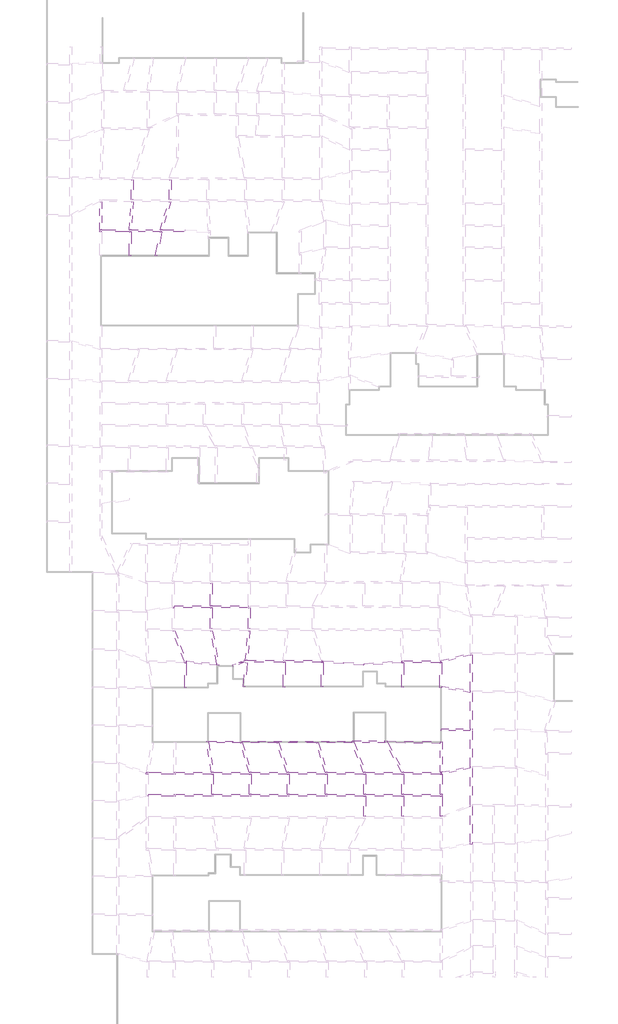
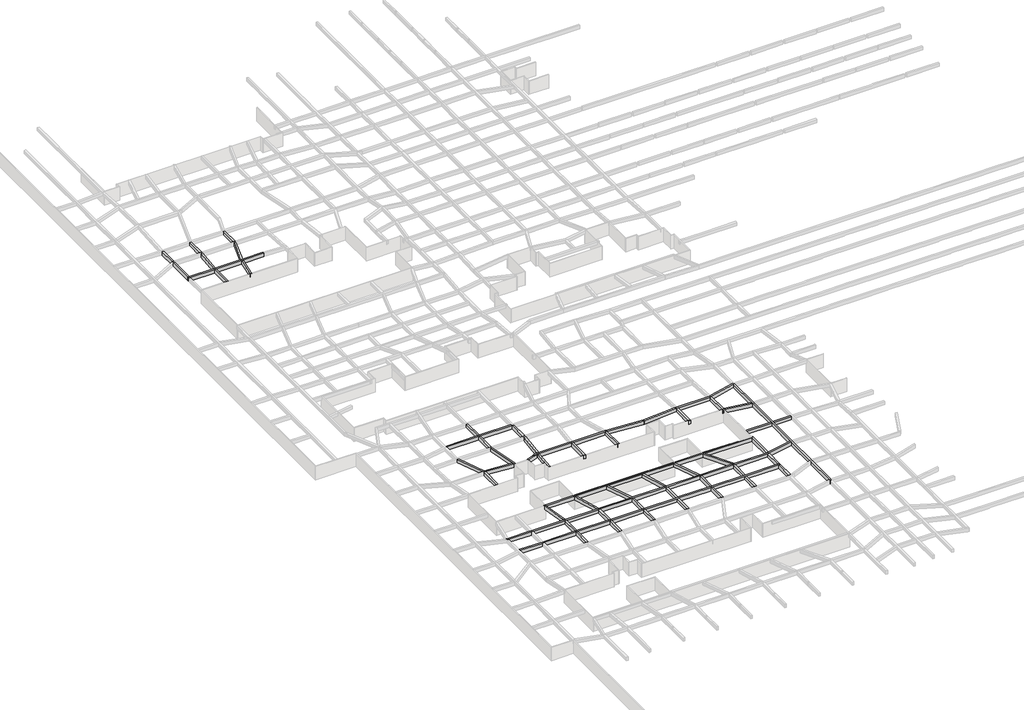
# One storey, part 15 of 45: 55 beams.
"""IFC4 building model written with IfcOpenShell, lengths in millimetres."""

from ifc_helpers import new_model, si_unit, frame, origin, place, context, project, spatial, polyline, outline, extrude, faceted_brep, element, save

model = new_model("IFC4")

# Units and contexts
model_context = context("Model", 3, world=origin())
ifc_project = project(units=[si_unit("LENGTHUNIT", "METRE", prefix="MILLI")], contexts=[model_context])

# Site, building, storey
site = spatial("IfcSite", under=ifc_project)
building = spatial("IfcBuilding", under=site)
storey = spatial("IfcBuildingStorey", under=building, Name="户型图", Elevation=0.0)

# Beams
placement = place(None, origin())
element("IfcBeam", 1, ObjectType="混凝土 - 矩形梁 : KL_beam", at=placement, inside=storey, context=model_context, shape_type="Brep", body=[
    faceted_brep([(-126607.5762912, -9543.8680223, 3300.0), (-126600.5942652, -9143.8680223, 3300.0), (-131304.5883974, -9143.8680223, 3300.0), (-131722.8651, -9143.8680223, 3300.0), (-137689.6115362, -9143.8680223, 3300.0), (-138090.5882954, -9143.8680223, 3300.0), (-143704.0852782, -9143.8680223, 3300.0), (-144104.0852782, -9143.8680223, 3300.0), (-144104.0852782, -9543.8680223, 3300.0), (-143704.0852782, -9543.8680223, 3300.0), (-138104.1004356, -9543.8680223, 3300.0), (-137704.1004356, -9543.8680223, 3300.0), (-131813.2236036, -9543.8680223, 3300.0), (-131407.0529588, -9543.8680223, 3300.0), (-126607.5762912, -9543.8680223, 2500.0), (-144104.0852782, -9543.8680223, 2500.0), (-143704.0852782, -9543.8680223, 2500.0), (-138104.1004356, -9543.8680223, 2500.0), (-137704.1004356, -9543.8680223, 2500.0), (-131813.2236036, -9543.8680223, 2500.0), (-131407.0529588, -9543.8680223, 2500.0), (-126600.5942652, -9143.8680223, 2500.0), (-144104.0852782, -9143.8680223, 2500.0), (-143704.0852782, -9143.8680223, 2500.0), (-138090.5882954, -9143.8680223, 2500.0), (-137689.6115362, -9143.8680223, 2500.0), (-131722.8651, -9143.8680223, 2500.0), (-131304.5883974, -9143.8680223, 2500.0)], [[[0, 1, 2, 3, 4, 5, 6, 7, 8, 9, 10, 11, 12, 13]], [[14, 0, 13, 12, 11, 10, 9, 8, 15, 16, 17, 18, 19, 20]], [[21, 14, 20, 19, 18, 17, 16, 15, 22, 23, 24, 25, 26, 27]], [[1, 21, 27, 26, 25, 24, 23, 22, 7, 6, 5, 4, 3, 2]], [[1, 0, 14, 21]], [[8, 7, 22, 15]]]),
])
element("IfcBeam", 2, ObjectType="混凝土 - 矩形梁 : KL_beam", at=placement, inside=storey, context=model_context, shape_type="Brep", body=[
    faceted_brep([(-143704.0852782, 1228.9879716, 3300.0), (-144104.0852782, 1242.9562794, 3300.0), (-144104.0852782, -2906.533538, 3300.0), (-143704.0852782, -2906.533538, 3300.0), (-143704.0852782, 1193.466462, 3300.0), (-143704.0852782, 1228.9879716, 2500.0), (-143704.0852782, -2906.533538, 2500.0), (-143704.0852782, 1193.466462, 2500.0), (-144104.0852782, 1242.9562794, 2500.0), (-144104.0852782, -2906.533538, 2500.0)], [[[0, 1, 2, 3, 4]], [[5, 0, 4, 3, 6, 7]], [[8, 5, 7, 6, 9]], [[1, 8, 9, 2]], [[1, 0, 5, 8]], [[3, 2, 9, 6]]]),
    faceted_brep([(-143704.0852782, -9143.8680223, 3300.0), (-144104.0852782, -9143.8680223, 3300.0), (-144104.0852782, -9143.8680223, 2500.0), (-143704.0852782, -9143.8680223, 2500.0), (-143704.0852782, -3306.533538, 3300.0), (-144104.0852782, -3306.533538, 3300.0), (-143704.0852782, -3306.533538, 2500.0), (-144104.0852782, -3306.533538, 2500.0)], [[[0, 1, 2, 3]], [[1, 0, 4, 5]], [[0, 3, 6, 4]], [[3, 2, 7, 6]], [[2, 1, 5, 7]], [[5, 4, 6, 7]]]),
])
element("IfcBeam", 3, ObjectType="混凝土 - 矩形梁 : KL_beam", at=placement, inside=storey, context=model_context, shape_type="SweptSolid", body=[
    extrude(outline(polyline([(-137682.4021047, -3306.533538), (-137281.4253454, -3306.533538), (-137689.6115362, -9143.8680223), (-138090.5882954, -9143.8680223), (-137682.4021047, -3306.533538)])), frame((0.0, 0.0, 2500.0), z_axis=(0.0, 0.0, 1.0), x_axis=(1.0, 0.0, 0.0)), (0.0, 0.0, 1.0), 800.0),
])
element("IfcBeam", 4, ObjectType="混凝土 - 矩形梁 : KL_beam", at=placement, inside=storey, context=model_context, shape_type="SweptSolid", body=[
    extrude(outline(polyline([(-137267.9283627, -2906.533538), (-137667.9283627, -2906.533538), (-137667.9283627, 1193.466462), (-137267.9283627, 1193.466462), (-137267.9283627, -2906.533538)])), frame((0.0, 0.0, 2500.0), z_axis=(0.0, 0.0, 1.0), x_axis=(1.0, 0.0, 0.0)), (0.0, 0.0, 1.0), 800.0),
])
element("IfcBeam", 5, ObjectType="混凝土 - 矩形梁 : KL_beam", at=placement, inside=storey, context=model_context, shape_type="SweptSolid", body=[
    extrude(outline(polyline([(-129467.9283627, -2906.533538), (-129867.9283627, -2906.533538), (-129867.9283627, 1193.466462), (-129467.9283627, 1193.466462), (-129467.9283627, -2906.533538)])), frame((0.0, 0.0, 2500.0), z_axis=(0.0, 0.0, 1.0), x_axis=(1.0, 0.0, 0.0)), (0.0, 0.0, 1.0), 800.0),
])
element("IfcBeam", 6, ObjectType="混凝土 - 矩形梁 : KL_beam", at=placement, inside=storey, context=model_context, shape_type="SweptSolid", body=[
    extrude(outline(polyline([(-129938.2128502, -3306.533538), (-129519.9361477, -3306.533538), (-131304.5883974, -9143.8680223), (-131722.8651, -9143.8680223), (-129938.2128502, -3306.533538)])), frame((0.0, 0.0, 2500.0), z_axis=(0.0, 0.0, 1.0), x_axis=(1.0, 0.0, 0.0)), (0.0, 0.0, 1.0), 800.0),
])
element("IfcBeam", 7, ObjectType="混凝土 - 矩形梁 : KL_beam", at=placement, inside=storey, context=model_context, shape_type="SweptSolid", body=[
    extrude(outline(polyline([(-137704.1004356, -14443.9764028), (-138104.1004356, -14443.9764028), (-138104.1004356, -9543.8680223), (-137704.1004356, -9543.8680223), (-137704.1004356, -14443.9764028)])), frame((0.0, 0.0, 2500.0), z_axis=(0.0, 0.0, 1.0), x_axis=(1.0, 0.0, 0.0)), (0.0, 0.0, 1.0), 800.0),
])
element("IfcBeam", 8, ObjectType="混凝土 - 矩形梁 : KL_beam", at=placement, inside=storey, context=model_context, shape_type="SweptSolid", body=[
    extrude(outline(polyline([(-132280.8818583, -14499.5979735), (-132674.8049595, -14430.1387024), (-131813.2236036, -9543.8680223), (-131407.0529588, -9543.8680223), (-132280.8818583, -14499.5979735)])), frame((0.0, 0.0, 2500.0), z_axis=(0.0, 0.0, 1.0), x_axis=(1.0, 0.0, 0.0)), (0.0, 0.0, 1.0), 800.0),
])
element("IfcBeam", 9, ObjectType="混凝土 - 矩形梁 : KL_beam", at=placement, inside=storey, context=model_context, shape_type="SweptSolid", body=[
    extrude(outline(polyline([(-121398.6286131, -81886.7344834), (-120998.6286131, -81886.7344834), (-120998.6286131, -86486.7344834), (-121398.6286131, -86486.7344834), (-121398.6286131, -81886.7344834)])), frame((0.0, 0.0, 2500.0), z_axis=(0.0, 0.0, 1.0), x_axis=(1.0, 0.0, 0.0)), (0.0, 0.0, 1.0), 800.0),
])
element("IfcBeam", 10, ObjectType="混凝土 - 矩形梁 : KL_beam", at=placement, inside=storey, context=model_context, shape_type="Brep", body=[
    faceted_brep([(-73810.3500115, -121175.3373066, 3300.0), (-73848.8656308, -120775.3373066, 3300.0), (-74029.6829415, -120775.3373066, 3300.0), (-81521.8778556, -120775.3373066, 3300.0), (-81979.2194827, -120775.3373066, 3300.0), (-89436.7705689, -120775.3373066, 3300.0), (-89865.2285663, -120775.3373066, 3300.0), (-97325.3650448, -120775.3373066, 3300.0), (-97742.8141387, -120775.3373066, 3300.0), (-105188.5127553, -120775.3373066, 3300.0), (-105613.1046235, -120775.3373066, 3300.0), (-112980.7461054, -120775.3373066, 3300.0), (-113398.1951993, -120775.3373066, 3300.0), (-120758.8698576, -120775.3373066, 3300.0), (-121163.8559079, -120775.3373066, 3300.0), (-128529.6078212, -120775.3373066, 3300.0), (-128929.6078212, -120775.3373066, 3300.0), (-134093.0297116, -120775.3373066, 3300.0), (-134498.6851719, -120775.3373066, 3300.0), (-134529.6078212, -120775.3373066, 3300.0), (-134529.6078212, -120958.5805757, 3300.0), (-134529.6078212, -121118.0480078, 3300.0), (-134529.6078212, -121175.3373066, 3300.0), (-134129.6078212, -121175.3373066, 3300.0), (-128929.6078212, -121175.3373066, 3300.0), (-128529.6078212, -121175.3373066, 3300.0), (-121129.6078212, -121175.3373066, 3300.0), (-120729.6078212, -121175.3373066, 3300.0), (-113329.6078212, -121175.3373066, 3300.0), (-112929.6078212, -121175.3373066, 3300.0), (-105529.6078212, -121175.3373066, 3300.0), (-105129.6078212, -121175.3373066, 3300.0), (-97674.2267606, -121175.3373066, 3300.0), (-97274.2267606, -121175.3373066, 3300.0), (-89774.2267606, -121175.3373066, 3300.0), (-89374.2267606, -121175.3373066, 3300.0), (-81974.2267606, -121175.3373066, 3300.0), (-81574.2267606, -121175.3373066, 3300.0), (-74074.2267606, -121175.3373066, 3300.0), (-73810.3500115, -121175.3373066, 2500.0), (-134529.6078212, -121175.3373066, 2500.0), (-134129.6078212, -121175.3373066, 2500.0), (-128929.6078212, -121175.3373066, 2500.0), (-128529.6078212, -121175.3373066, 2500.0), (-121129.6078212, -121175.3373066, 2500.0), (-120729.6078212, -121175.3373066, 2500.0), (-113329.6078212, -121175.3373066, 2500.0), (-112929.6078212, -121175.3373066, 2500.0), (-105529.6078212, -121175.3373066, 2500.0), (-105129.6078212, -121175.3373066, 2500.0), (-97674.2267606, -121175.3373066, 2500.0), (-97274.2267606, -121175.3373066, 2500.0), (-89774.2267606, -121175.3373066, 2500.0), (-89374.2267606, -121175.3373066, 2500.0), (-81974.2267606, -121175.3373066, 2500.0), (-81574.2267606, -121175.3373066, 2500.0), (-74074.2267606, -121175.3373066, 2500.0), (-73848.8656308, -120775.3373066, 2500.0), (-134529.6078212, -121118.0480078, 2500.0), (-134529.6078212, -120958.5805757, 2500.0), (-134529.6078212, -120775.3373066, 2500.0), (-134498.6851719, -120775.3373066, 2500.0), (-134093.0297116, -120775.3373066, 2500.0), (-128929.6078212, -120775.3373066, 2500.0), (-128529.6078212, -120775.3373066, 2500.0), (-121163.8559079, -120775.3373066, 2500.0), (-120758.8698576, -120775.3373066, 2500.0), (-113398.1951993, -120775.3373066, 2500.0), (-112980.7461054, -120775.3373066, 2500.0), (-105613.1046235, -120775.3373066, 2500.0), (-105188.5127553, -120775.3373066, 2500.0), (-97742.8141387, -120775.3373066, 2500.0), (-97325.3650448, -120775.3373066, 2500.0), (-89865.2285663, -120775.3373066, 2500.0), (-89436.7705689, -120775.3373066, 2500.0), (-81979.2194827, -120775.3373066, 2500.0), (-81521.8778556, -120775.3373066, 2500.0), (-74029.6829415, -120775.3373066, 2500.0)], [[[0, 1, 2, 3, 4, 5, 6, 7, 8, 9, 10, 11, 12, 13, 14, 15, 16, 17, 18, 19, 20, 21, 22, 23, 24, 25, 26, 27, 28, 29, 30, 31, 32, 33, 34, 35, 36, 37, 38]], [[39, 0, 38, 37, 36, 35, 34, 33, 32, 31, 30, 29, 28, 27, 26, 25, 24, 23, 22, 40, 41, 42, 43, 44, 45, 46, 47, 48, 49, 50, 51, 52, 53, 54, 55, 56]], [[57, 39, 56, 55, 54, 53, 52, 51, 50, 49, 48, 47, 46, 45, 44, 43, 42, 41, 40, 58, 59, 60, 61, 62, 63, 64, 65, 66, 67, 68, 69, 70, 71, 72, 73, 74, 75, 76, 77]], [[1, 57, 77, 76, 75, 74, 73, 72, 71, 70, 69, 68, 67, 66, 65, 64, 63, 62, 61, 60, 19, 18, 17, 16, 15, 14, 13, 12, 11, 10, 9, 8, 7, 6, 5, 4, 3, 2]], [[22, 21, 20, 19, 60, 59, 58, 40]], [[1, 0, 39, 57]]]),
])
element("IfcBeam", 11, ObjectType="混凝土 - 矩形梁 : KL_beam", at=placement, inside=storey, context=model_context, shape_type="Brep", body=[
    faceted_brep([(-73674.2267606, -125746.3030805, 3300.0), (-73674.2267606, -125346.3030805, 3300.0), (-74074.2267606, -125346.3030805, 3300.0), (-81574.2267606, -125346.3030805, 3300.0), (-81974.2267606, -125346.3030805, 3300.0), (-89374.2267606, -125346.3030805, 3300.0), (-89774.2267606, -125346.3030805, 3300.0), (-97274.2267606, -125346.3030805, 3300.0), (-97674.2267606, -125346.3030805, 3300.0), (-105129.6078212, -125346.3030805, 3300.0), (-105529.6078212, -125346.3030805, 3300.0), (-112929.6078212, -125346.3030805, 3300.0), (-113329.6078212, -125346.3030805, 3300.0), (-120729.6078212, -125346.3030805, 3300.0), (-121129.6078212, -125346.3030805, 3300.0), (-128529.6078212, -125346.3030805, 3300.0), (-128929.6078212, -125346.3030805, 3300.0), (-134129.6078212, -125346.3030805, 3300.0), (-134129.6078212, -125746.3030805, 3300.0), (-128929.6078212, -125746.3030805, 3300.0), (-128529.6078212, -125746.3030805, 3300.0), (-121129.6078212, -125746.3030805, 3300.0), (-120729.6078212, -125746.3030805, 3300.0), (-113329.6078212, -125746.3030805, 3300.0), (-112929.6078212, -125746.3030805, 3300.0), (-105529.6078212, -125746.3030805, 3300.0), (-105129.6078212, -125746.3030805, 3300.0), (-97674.2267606, -125746.3030805, 3300.0), (-97274.2267606, -125746.3030805, 3300.0), (-89774.2267606, -125746.3030805, 3300.0), (-89374.2267606, -125746.3030805, 3300.0), (-81974.2267606, -125746.3030805, 3300.0), (-81574.2267606, -125746.3030805, 3300.0), (-74074.2267606, -125746.3030805, 3300.0), (-73674.2267606, -125746.3030805, 2500.0), (-134129.6078212, -125746.3030805, 2500.0), (-128929.6078212, -125746.3030805, 2500.0), (-128529.6078212, -125746.3030805, 2500.0), (-121129.6078212, -125746.3030805, 2500.0), (-120729.6078212, -125746.3030805, 2500.0), (-113329.6078212, -125746.3030805, 2500.0), (-112929.6078212, -125746.3030805, 2500.0), (-105529.6078212, -125746.3030805, 2500.0), (-105129.6078212, -125746.3030805, 2500.0), (-97674.2267606, -125746.3030805, 2500.0), (-97274.2267606, -125746.3030805, 2500.0), (-89774.2267606, -125746.3030805, 2500.0), (-89374.2267606, -125746.3030805, 2500.0), (-81974.2267606, -125746.3030805, 2500.0), (-81574.2267606, -125746.3030805, 2500.0), (-74074.2267606, -125746.3030805, 2500.0), (-73674.2267606, -125346.3030805, 2500.0), (-134129.6078212, -125346.3030805, 2500.0), (-128929.6078212, -125346.3030805, 2500.0), (-128529.6078212, -125346.3030805, 2500.0), (-121129.6078212, -125346.3030805, 2500.0), (-120729.6078212, -125346.3030805, 2500.0), (-113329.6078212, -125346.3030805, 2500.0), (-112929.6078212, -125346.3030805, 2500.0), (-105529.6078212, -125346.3030805, 2500.0), (-105129.6078212, -125346.3030805, 2500.0), (-97674.2267606, -125346.3030805, 2500.0), (-97274.2267606, -125346.3030805, 2500.0), (-89774.2267606, -125346.3030805, 2500.0), (-89374.2267606, -125346.3030805, 2500.0), (-81974.2267606, -125346.3030805, 2500.0), (-81574.2267606, -125346.3030805, 2500.0), (-74074.2267606, -125346.3030805, 2500.0)], [[[0, 1, 2, 3, 4, 5, 6, 7, 8, 9, 10, 11, 12, 13, 14, 15, 16, 17, 18, 19, 20, 21, 22, 23, 24, 25, 26, 27, 28, 29, 30, 31, 32, 33]], [[34, 0, 33, 32, 31, 30, 29, 28, 27, 26, 25, 24, 23, 22, 21, 20, 19, 18, 35, 36, 37, 38, 39, 40, 41, 42, 43, 44, 45, 46, 47, 48, 49, 50]], [[51, 34, 50, 49, 48, 47, 46, 45, 44, 43, 42, 41, 40, 39, 38, 37, 36, 35, 52, 53, 54, 55, 56, 57, 58, 59, 60, 61, 62, 63, 64, 65, 66, 67]], [[1, 51, 67, 66, 65, 64, 63, 62, 61, 60, 59, 58, 57, 56, 55, 54, 53, 52, 17, 16, 15, 14, 13, 12, 11, 10, 9, 8, 7, 6, 5, 4, 3, 2]], [[18, 17, 52, 35]], [[1, 0, 34, 51]]]),
])
element("IfcBeam", 12, ObjectType="混凝土 - 矩形梁 : KL_beam", at=placement, inside=storey, context=model_context, shape_type="SweptSolid", body=[
    extrude(outline(polyline([(-121129.6078212, -121175.3373066), (-120729.6078212, -121175.3373066), (-120729.6078212, -125346.3030805), (-121129.6078212, -125346.3030805), (-121129.6078212, -121175.3373066)])), frame((0.0, 0.0, 2500.0), z_axis=(0.0, 0.0, 1.0), x_axis=(1.0, 0.0, 0.0)), (0.0, 0.0, 1.0), 800.0),
    extrude(outline(polyline([(-120729.6078212, -129869.3244435), (-121129.6078212, -129869.3244435), (-121129.6078212, -125746.3030805), (-120729.6078212, -125746.3030805), (-120729.6078212, -129869.3244435)])), frame((0.0, 0.0, 2500.0), z_axis=(0.0, 0.0, 1.0), x_axis=(1.0, 0.0, 0.0)), (0.0, 0.0, 1.0), 800.0),
])
element("IfcBeam", 13, ObjectType="混凝土 - 矩形梁 : KL_beam", at=placement, inside=storey, context=model_context, shape_type="SweptSolid", body=[
    extrude(outline(polyline([(-113329.6078212, -121175.3373066), (-112929.6078212, -121175.3373066), (-112929.6078212, -125346.3030805), (-113329.6078212, -125346.3030805), (-113329.6078212, -121175.3373066)])), frame((0.0, 0.0, 2500.0), z_axis=(0.0, 0.0, 1.0), x_axis=(1.0, 0.0, 0.0)), (0.0, 0.0, 1.0), 800.0),
    extrude(outline(polyline([(-112929.6078212, -129869.3244435), (-113329.6078212, -129869.3244435), (-113329.6078212, -125746.3030805), (-112929.6078212, -125746.3030805), (-112929.6078212, -129869.3244435)])), frame((0.0, 0.0, 2500.0), z_axis=(0.0, 0.0, 1.0), x_axis=(1.0, 0.0, 0.0)), (0.0, 0.0, 1.0), 800.0),
])
element("IfcBeam", 14, ObjectType="混凝土 - 矩形梁 : KL_beam", at=placement, inside=storey, context=model_context, shape_type="SweptSolid", body=[
    extrude(outline(polyline([(-105529.6078212, -121175.3373066), (-105129.6078212, -121175.3373066), (-105129.6078212, -125346.3030805), (-105529.6078212, -125346.3030805), (-105529.6078212, -121175.3373066)])), frame((0.0, 0.0, 2500.0), z_axis=(0.0, 0.0, 1.0), x_axis=(1.0, 0.0, 0.0)), (0.0, 0.0, 1.0), 800.0),
    extrude(outline(polyline([(-105129.6078212, -129869.3244435), (-105529.6078212, -129869.3244435), (-105529.6078212, -125746.3030805), (-105129.6078212, -125746.3030805), (-105129.6078212, -129869.3244435)])), frame((0.0, 0.0, 2500.0), z_axis=(0.0, 0.0, 1.0), x_axis=(1.0, 0.0, 0.0)), (0.0, 0.0, 1.0), 800.0),
])
element("IfcBeam", 15, ObjectType="混凝土 - 矩形梁 : KL_beam", at=placement, inside=storey, context=model_context, shape_type="Brep", body=[
    faceted_brep([(-113598.6286131, -86886.7344834, 3300.0), (-113598.6286131, -86486.7344834, 3300.0), (-120998.6286131, -86486.7344834, 3300.0), (-121398.6286131, -86486.7344834, 3300.0), (-128818.6286131, -86486.7344834, 3300.0), (-128818.6286131, -86854.5544096, 3300.0), (-129001.1308804, -86886.7344834, 3300.0), (-128818.6286131, -86886.7344834, 3300.0), (-121398.6286131, -86886.7344834, 3300.0), (-120998.6286131, -86886.7344834, 3300.0), (-113598.6286131, -86886.7344834, 2500.0), (-129001.1308804, -86886.7344834, 2500.0), (-128818.6286131, -86886.7344834, 2500.0), (-121398.6286131, -86886.7344834, 2500.0), (-120998.6286131, -86886.7344834, 2500.0), (-113598.6286131, -86486.7344834, 2500.0), (-128818.6286131, -86854.5544096, 2500.0), (-128818.6286131, -86486.7344834, 2500.0), (-121398.6286131, -86486.7344834, 2500.0), (-120998.6286131, -86486.7344834, 2500.0)], [[[0, 1, 2, 3, 4, 5, 6, 7, 8, 9]], [[10, 0, 9, 8, 7, 6, 11, 12, 13, 14]], [[15, 10, 14, 13, 12, 11, 16, 17, 18, 19]], [[1, 15, 19, 18, 17, 4, 3, 2]], [[1, 0, 10, 15]], [[16, 5, 4, 17]], [[5, 16, 11, 6]]]),
])
element("IfcBeam", 16, ObjectType="混凝土 - 矩形梁 : KL_beam", at=placement, inside=storey, context=model_context, shape_type="SweptSolid", body=[
    extrude(outline(polyline([(-121398.6286131, -86886.7344834), (-120998.6286131, -86886.7344834), (-120998.6286131, -91241.7669719), (-121398.6286131, -91241.7669719), (-121398.6286131, -86886.7344834)])), frame((0.0, 0.0, 2500.0), z_axis=(0.0, 0.0, 1.0), x_axis=(1.0, 0.0, 0.0)), (0.0, 0.0, 1.0), 800.0),
])
element("IfcBeam", 17, ObjectType="混凝土 - 矩形梁 : KL_beam", at=placement, inside=storey, context=model_context, shape_type="Brep", body=[
    faceted_brep([(-126624.1724793, -98237.624084, 3300.0), (-126600.2797743, -98228.4525338, 3300.0), (-126250.7403087, -98094.2769042, 3300.0), (-126344.786832, -97849.2773349, 3300.0), (-128727.6268074, -91641.7669719, 3300.0), (-129156.0848049, -91641.7669719, 3300.0), (-126777.7180933, -97837.624084, 3300.0), (-126624.1724793, -98237.624084, 2500.0), (-129156.0848049, -91641.7669719, 2500.0), (-126777.7180933, -97837.624084, 2500.0), (-126250.7403087, -98094.2769042, 2500.0), (-126600.2797743, -98228.4525338, 2500.0), (-128727.6268074, -91641.7669719, 2500.0), (-126344.786832, -97849.2773349, 2500.0)], [[[0, 1, 2, 3, 4, 5, 6]], [[7, 0, 6, 5, 8, 9]], [[10, 11, 7, 9, 8, 12, 13]], [[2, 10, 13, 12, 4, 3]], [[5, 4, 12, 8]], [[2, 1, 0, 7, 11, 10]]]),
])
element("IfcBeam", 18, ObjectType="混凝土 - 矩形梁 : KL_beam", at=placement, inside=storey, context=model_context, shape_type="Brep", body=[
    faceted_brep([(-119970.4261366, -98808.4895679, 3300.0), (-119577.7752632, -98732.1659698, 3300.0), (-120956.0092123, -91641.7669719, 3300.0), (-121363.4958903, -91641.7669719, 3300.0), (-120049.8255327, -98400.0150859, 3300.0), (-119970.4261366, -98808.4895679, 2500.0), (-121363.4958903, -91641.7669719, 2500.0), (-120049.8255327, -98400.0150859, 2500.0), (-119577.7752632, -98732.1659698, 2500.0), (-120956.0092123, -91641.7669719, 2500.0)], [[[0, 1, 2, 3, 4]], [[5, 0, 4, 3, 6, 7]], [[8, 5, 7, 6, 9]], [[1, 8, 9, 2]], [[3, 2, 9, 6]], [[1, 0, 5, 8]]]),
])
element("IfcBeam", 19, ObjectType="混凝土 - 矩形梁 : KL_beam", at=placement, inside=storey, context=model_context, shape_type="Brep", body=[
    faceted_brep([(-98302.2751608, -98176.6407423, 3300.0), (-98287.4686336, -97776.6407423, 3300.0), (-98563.7893521, -97776.6407423, 3300.0), (-105946.1060855, -97776.6407423, 3300.0), (-106347.6340205, -97776.6407423, 3300.0), (-113752.0942854, -97776.6407423, 3300.0), (-114153.6222204, -97776.6407423, 3300.0), (-114450.8945963, -97776.6407423, 3300.0), (-115492.9302222, -98176.6407423, 3300.0), (-114376.7589783, -98176.6407423, 3300.0), (-106364.3677857, -98176.6407423, 3300.0), (-105964.3677857, -98176.6407423, 3300.0), (-98494.8718972, -98176.6407423, 3300.0), (-98287.4686336, -97776.6407423, 2500.0), (-98563.7893521, -97776.6407423, 2500.0), (-105946.1060855, -97776.6407423, 2500.0), (-106347.6340205, -97776.6407423, 2500.0), (-113752.0942854, -97776.6407423, 2500.0), (-114153.6222204, -97776.6407423, 2500.0), (-114450.8945963, -97776.6407423, 2500.0), (-98302.2751608, -98176.6407423, 2500.0), (-98494.8718972, -98176.6407423, 2500.0), (-105964.3677857, -98176.6407423, 2500.0), (-106364.3677857, -98176.6407423, 2500.0), (-114376.7589783, -98176.6407423, 2500.0), (-115492.9302222, -98176.6407423, 2500.0)], [[[0, 1, 2, 3, 4, 5, 6, 7, 8, 9, 10, 11, 12]], [[1, 13, 14, 15, 16, 17, 18, 19, 7, 6, 5, 4, 3, 2]], [[13, 20, 21, 22, 23, 24, 25, 19, 18, 17, 16, 15, 14]], [[20, 0, 12, 11, 10, 9, 8, 25, 24, 23, 22, 21]], [[0, 20, 13, 1]], [[8, 7, 19, 25]]]),
])
element("IfcBeam", 20, ObjectType="混凝土 - 矩形梁 : KL_beam", at=placement, inside=storey, context=model_context, shape_type="Brep", body=[
    faceted_brep([(-73955.7721969, -98206.5978244, 3300.0), (-74005.7852131, -97806.5978244, 3300.0), (-74190.6863209, -97806.5978244, 3300.0), (-81590.2186825, -97806.5978244, 3300.0), (-81990.6863209, -97806.5978244, 3300.0), (-81989.968125, -97821.4460968, 3300.0), (-81980.778705, -98011.431897, 3300.0), (-81971.3387275, -98206.5978244, 3300.0), (-81580.778705, -98206.5978244, 3300.0), (-74180.6241203, -98206.5978244, 3300.0), (-73955.7721969, -98206.5978244, 2500.0), (-81971.3387275, -98206.5978244, 2500.0), (-81580.778705, -98206.5978244, 2500.0), (-74180.6241203, -98206.5978244, 2500.0), (-74005.7852131, -97806.5978244, 2500.0), (-81980.778705, -98011.431897, 2500.0), (-81989.968125, -97821.4460968, 2500.0), (-81990.6863209, -97806.5978244, 2500.0), (-81590.2186825, -97806.5978244, 2500.0), (-74190.6863209, -97806.5978244, 2500.0)], [[[0, 1, 2, 3, 4, 5, 6, 7, 8, 9]], [[10, 0, 9, 8, 7, 11, 12, 13]], [[14, 10, 13, 12, 11, 15, 16, 17, 18, 19]], [[1, 14, 19, 18, 17, 4, 3, 2]], [[1, 0, 10, 14]], [[7, 6, 5, 4, 17, 16, 15, 11]]]),
])
element("IfcBeam", 21, ObjectType="混凝土 - 矩形梁 : KL_beam", at=placement, inside=storey, context=model_context, shape_type="Brep", body=[
    faceted_brep([(-67725.9320986, -96211.286122, 3300.0), (-67830.7823984, -96237.9219218, 3300.0), (-73792.8353015, -97752.5007811, 3300.0), (-74005.7852131, -97806.5978244, 3300.0), (-73955.7721969, -98206.5978244, 3300.0), (-73780.6241203, -98162.1038257, 3300.0), (-67830.7823984, -96650.6270517, 3300.0), (-67675.9190824, -96611.286122, 3300.0), (-73955.7721969, -98206.5978244, 2500.0), (-73780.6241203, -98162.1038257, 2500.0), (-67830.7823984, -96650.6270517, 2500.0), (-67675.9190824, -96611.286122, 2500.0), (-74005.7852131, -97806.5978244, 2500.0), (-73792.8353015, -97752.5007811, 2500.0), (-67830.7823984, -96237.9219218, 2500.0), (-67725.9320986, -96211.286122, 2500.0)], [[[0, 1, 2, 3, 4, 5, 6, 7]], [[7, 6, 5, 4, 8, 9, 10, 11]], [[11, 10, 9, 8, 12, 13, 14, 15]], [[3, 2, 1, 0, 15, 14, 13, 12]], [[0, 7, 11, 15]], [[3, 12, 8, 4]]]),
])
element("IfcBeam", 22, ObjectType="混凝土 - 矩形梁 : KL_beam", at=placement, inside=storey, context=model_context, shape_type="Brep", body=[
    faceted_brep([(-67430.7823984, -96611.286122, 3300.0), (-67675.9190824, -96611.286122, 3300.0), (-67830.7823984, -96650.6270517, 3300.0), (-67830.7823984, -103977.1522138, 3300.0), (-67830.7823984, -104382.1285271, 3300.0), (-67830.7823984, -111828.4346923, 3300.0), (-67830.7823984, -112228.4346923, 3300.0), (-67830.7823984, -119605.5404275, 3300.0), (-67830.7823984, -120013.0271055, 3300.0), (-67830.7823984, -127430.3404481, 3300.0), (-67830.7823984, -127861.7543451, 3300.0), (-67830.7823984, -135248.1884022, 3300.0), (-67830.7823984, -135656.5378646, 3300.0), (-67764.0267672, -135642.8272555, 3300.0), (-67610.4560354, -135611.286122, 3300.0), (-67430.7823984, -135574.3838418, 3300.0), (-67430.7823984, -135211.286122, 3300.0), (-67430.7823984, -127765.3480623, 3300.0), (-67430.7823984, -127365.3480623, 3300.0), (-67430.7823984, -119970.4077047, 3300.0), (-67430.7823984, -119570.4077047, 3300.0), (-67430.7823984, -112228.4346923, 3300.0), (-67430.7823984, -111828.4346923, 3300.0), (-67430.7823984, -104411.286122, 3300.0), (-67430.7823984, -104011.286122, 3300.0), (-67830.7823984, -96650.6270517, 2500.0), (-67830.7823984, -103977.1522138, 2500.0), (-67830.7823984, -104382.1285271, 2500.0), (-67830.7823984, -111828.4346923, 2500.0), (-67830.7823984, -112228.4346923, 2500.0), (-67830.7823984, -119605.5404275, 2500.0), (-67830.7823984, -120013.0271055, 2500.0), (-67830.7823984, -127430.3404481, 2500.0), (-67830.7823984, -127861.7543451, 2500.0), (-67830.7823984, -135248.1884022, 2500.0), (-67830.7823984, -135656.5378646, 2500.0), (-67675.9190824, -96611.286122, 2500.0), (-67430.7823984, -96611.286122, 2500.0), (-67430.7823984, -104011.286122, 2500.0), (-67430.7823984, -104411.286122, 2500.0), (-67430.7823984, -111828.4346923, 2500.0), (-67430.7823984, -112228.4346923, 2500.0), (-67430.7823984, -119570.4077047, 2500.0), (-67430.7823984, -119970.4077047, 2500.0), (-67430.7823984, -127365.3480623, 2500.0), (-67430.7823984, -127765.3480623, 2500.0), (-67430.7823984, -135211.286122, 2500.0), (-67430.7823984, -135574.3838418, 2500.0), (-67610.4560354, -135611.286122, 2500.0), (-67764.0267672, -135642.8272555, 2500.0)], [[[0, 1, 2, 3, 4, 5, 6, 7, 8, 9, 10, 11, 12, 13, 14, 15, 16, 17, 18, 19, 20, 21, 22, 23, 24]], [[2, 25, 26, 27, 28, 29, 30, 31, 32, 33, 34, 35, 12, 11, 10, 9, 8, 7, 6, 5, 4, 3]], [[36, 37, 38, 39, 40, 41, 42, 43, 44, 45, 46, 47, 48, 49, 35, 34, 33, 32, 31, 30, 29, 28, 27, 26, 25]], [[37, 0, 24, 23, 22, 21, 20, 19, 18, 17, 16, 15, 47, 46, 45, 44, 43, 42, 41, 40, 39, 38]], [[1, 0, 37, 36]], [[2, 1, 36, 25]], [[15, 14, 13, 12, 35, 49, 48, 47]]]),
])
element("IfcBeam", 23, ObjectType="混凝土 - 矩形梁 : KL_beam", at=placement, inside=storey, context=model_context, shape_type="Brep", body=[
    faceted_brep([(-73848.8656308, -120775.3373066, 3300.0), (-73810.3500115, -121175.3373066, 3300.0), (-73674.2267606, -121148.877627, 3300.0), (-67830.7823984, -120013.0271055, 3300.0), (-67830.7823984, -119605.5404275, 3300.0), (-73629.6829415, -120732.7325077, 3300.0), (-73810.3500115, -121175.3373066, 2500.0), (-73674.2267606, -121148.877627, 2500.0), (-67830.7823984, -120013.0271055, 2500.0), (-73848.8656308, -120775.3373066, 2500.0), (-73629.6829415, -120732.7325077, 2500.0), (-67830.7823984, -119605.5404275, 2500.0)], [[[0, 1, 2, 3, 4, 5]], [[1, 6, 7, 8, 3, 2]], [[6, 9, 10, 11, 8, 7]], [[9, 0, 5, 4, 11, 10]], [[0, 9, 6, 1]], [[4, 3, 8, 11]]]),
])
element("IfcBeam", 24, ObjectType="混凝土 - 矩形梁 : KL_beam", at=placement, inside=storey, context=model_context, shape_type="SweptSolid", body=[
    extrude(outline(polyline([(-97674.2267606, -121175.3373066), (-97274.2267606, -121175.3373066), (-97274.2267606, -125346.3030805), (-97674.2267606, -125346.3030805), (-97674.2267606, -121175.3373066)])), frame((0.0, 0.0, 2500.0), z_axis=(0.0, 0.0, 1.0), x_axis=(1.0, 0.0, 0.0)), (0.0, 0.0, 1.0), 800.0),
    extrude(outline(polyline([(-97274.2267606, -129869.3244435), (-97674.2267606, -129869.3244435), (-97674.2267606, -125746.3030805), (-97274.2267606, -125746.3030805), (-97274.2267606, -129869.3244435)])), frame((0.0, 0.0, 2500.0), z_axis=(0.0, 0.0, 1.0), x_axis=(1.0, 0.0, 0.0)), (0.0, 0.0, 1.0), 800.0),
])
element("IfcBeam", 25, ObjectType="混凝土 - 矩形梁 : KL_beam", at=placement, inside=storey, context=model_context, shape_type="Brep", body=[
    faceted_brep([(-91909.5094207, -114333.6323638, 3300.0), (-91968.3714548, -114356.2273817, 3300.0), (-92282.9415913, -114476.9795436, 3300.0), (-92175.7483894, -114756.2273817, 3300.0), (-89865.2285663, -120775.3373066, 3300.0), (-89436.7705689, -120775.3373066, 3300.0), (-91755.9638067, -114733.6323638, 3300.0), (-91909.5094207, -114333.6323638, 2500.0), (-89436.7705689, -120775.3373066, 2500.0), (-91755.9638067, -114733.6323638, 2500.0), (-92282.9415913, -114476.9795436, 2500.0), (-91968.3714548, -114356.2273817, 2500.0), (-89865.2285663, -120775.3373066, 2500.0), (-92175.7483894, -114756.2273817, 2500.0)], [[[0, 1, 2, 3, 4, 5, 6]], [[7, 0, 6, 5, 8, 9]], [[10, 11, 7, 9, 8, 12, 13]], [[2, 10, 13, 12, 4, 3]], [[5, 4, 12, 8]], [[2, 1, 0, 7, 11, 10]]]),
])
element("IfcBeam", 26, ObjectType="混凝土 - 矩形梁 : KL_beam", at=placement, inside=storey, context=model_context, shape_type="Brep", body=[
    faceted_brep([(-85092.5732122, -114333.6323638, 3300.0), (-85549.9148393, -114333.6323638, 3300.0), (-85328.1912188, -114733.6323638, 3300.0), (-81979.2194827, -120775.3373066, 3300.0), (-81521.8778556, -120775.3373066, 3300.0), (-84868.4375117, -114737.9838712, 3300.0), (-85091.7243385, -114335.1637725, 3300.0), (-85092.5732122, -114333.6323638, 2500.0), (-81521.8778556, -120775.3373066, 2500.0), (-84868.4375117, -114737.9838712, 2500.0), (-85091.7243385, -114335.1637725, 2500.0), (-85549.9148393, -114333.6323638, 2500.0), (-81979.2194827, -120775.3373066, 2500.0), (-85328.1912188, -114733.6323638, 2500.0)], [[[0, 1, 2, 3, 4, 5, 6]], [[7, 0, 6, 5, 4, 8, 9, 10]], [[11, 7, 10, 9, 8, 12, 13]], [[1, 11, 13, 12, 3, 2]], [[4, 3, 12, 8]], [[1, 0, 7, 11]]]),
])
element("IfcBeam", 27, ObjectType="混凝土 - 矩形梁 : KL_beam", at=placement, inside=storey, context=model_context, shape_type="Brep", body=[
    faceted_brep([(-74029.6829415, -120775.3373066, 3300.0), (-73848.8656308, -120775.3373066, 3300.0), (-73629.6829415, -120732.7325077, 3300.0), (-73629.6829415, -114478.3270492, 3300.0), (-74029.6829415, -114473.3309662, 3300.0), (-74029.6829415, -114873.362166, 3300.0), (-73629.6829415, -114478.3270492, 2500.0), (-73629.6829415, -120732.7325077, 2500.0), (-73848.8656308, -120775.3373066, 2500.0), (-74029.6829415, -120775.3373066, 2500.0), (-74029.6829415, -114873.362166, 2500.0), (-74029.6829415, -114473.3309662, 2500.0)], [[[0, 1, 2, 3, 4, 5]], [[6, 3, 2, 7]], [[8, 9, 10, 11, 6, 7]], [[9, 0, 5, 4, 11, 10]], [[1, 0, 9, 8]], [[2, 1, 8, 7]], [[4, 3, 6, 11]]]),
])
element("IfcBeam", 28, ObjectType="混凝土 - 矩形梁 : KL_beam", at=placement, inside=storey, context=model_context, shape_type="Brep", body=[
    faceted_brep([(-74074.2267606, -125346.3030805, 3300.0), (-73674.2267606, -125346.3030805, 3300.0), (-73674.2267606, -121148.877627, 3300.0), (-73810.3500115, -121175.3373066, 3300.0), (-74029.6829415, -121175.3373066, 3300.0), (-74074.2267606, -121175.3373066, 3300.0), (-73674.2267606, -125346.3030805, 2500.0), (-73674.2267606, -121148.877627, 2500.0), (-74074.2267606, -125346.3030805, 2500.0), (-74074.2267606, -121175.3373066, 2500.0), (-74029.6829415, -121175.3373066, 2500.0), (-73810.3500115, -121175.3373066, 2500.0)], [[[0, 1, 2, 3, 4, 5]], [[1, 6, 7, 2]], [[6, 8, 9, 10, 11, 7]], [[8, 0, 5, 9]], [[1, 0, 8, 6]], [[9, 5, 4, 3, 11, 10]], [[3, 2, 7, 11]]]),
])
element("IfcBeam", 29, ObjectType="混凝土 - 矩形梁 : KL_beam", at=placement, inside=storey, context=model_context, shape_type="SweptSolid", body=[
    extrude(outline(polyline([(-81974.2267606, -121175.3373066), (-81574.2267606, -121175.3373066), (-81574.2267606, -125346.3030805), (-81974.2267606, -125346.3030805), (-81974.2267606, -121175.3373066)])), frame((0.0, 0.0, 2500.0), z_axis=(0.0, 0.0, 1.0), x_axis=(1.0, 0.0, 0.0)), (0.0, 0.0, 1.0), 800.0),
])
element("IfcBeam", 30, ObjectType="混凝土 - 矩形梁 : KL_beam", at=placement, inside=storey, context=model_context, shape_type="SweptSolid", body=[
    extrude(outline(polyline([(-89774.2267606, -121175.3373066), (-89374.2267606, -121175.3373066), (-89374.2267606, -125346.3030805), (-89774.2267606, -125346.3030805), (-89774.2267606, -121175.3373066)])), frame((0.0, 0.0, 2500.0), z_axis=(0.0, 0.0, 1.0), x_axis=(1.0, 0.0, 0.0)), (0.0, 0.0, 1.0), 800.0),
])
element("IfcBeam", 31, ObjectType="混凝土 - 矩形梁 : KL_beam", at=placement, inside=storey, context=model_context, shape_type="SweptSolid", body=[
    extrude(outline(polyline([(-89774.2267606, -125746.3030805), (-89374.2267606, -125746.3030805), (-89374.2267606, -129869.3244435), (-89774.2267606, -129869.3244435), (-89774.2267606, -125746.3030805)])), frame((0.0, 0.0, 2500.0), z_axis=(0.0, 0.0, 1.0), x_axis=(1.0, 0.0, 0.0)), (0.0, 0.0, 1.0), 800.0),
])
element("IfcBeam", 32, ObjectType="混凝土 - 矩形梁 : KL_beam", at=placement, inside=storey, context=model_context, shape_type="SweptSolid", body=[
    extrude(outline(polyline([(-81974.2267606, -125746.3030805), (-81574.2267606, -125746.3030805), (-81574.2267606, -129869.3244435), (-81974.2267606, -129869.3244435), (-81974.2267606, -125746.3030805)])), frame((0.0, 0.0, 2500.0), z_axis=(0.0, 0.0, 1.0), x_axis=(1.0, 0.0, 0.0)), (0.0, 0.0, 1.0), 800.0),
])
element("IfcBeam", 33, ObjectType="混凝土 - 矩形梁 : KL_beam", at=placement, inside=storey, context=model_context, shape_type="SweptSolid", body=[
    extrude(outline(polyline([(-74074.2267606, -125746.3030805), (-73674.2267606, -125746.3030805), (-73674.2267606, -129791.2452196), (-73867.4796211, -129869.3244435), (-74074.2267606, -129869.3244435), (-74074.2267606, -125746.3030805)])), frame((0.0, 0.0, 2500.0), z_axis=(0.0, 0.0, 1.0), x_axis=(1.0, 0.0, 0.0)), (0.0, 0.0, 1.0), 800.0),
])
element("IfcBeam", 34, ObjectType="混凝土 - 矩形梁 : KL_beam", at=placement, inside=storey, context=model_context, shape_type="SweptSolid", body=[
    extrude(outline(polyline([(-73829.6762806, -112228.4346923), (-73829.6762806, -111828.4346923), (-67830.7823984, -111828.4346923), (-67830.7823984, -112228.4346923), (-73829.6762806, -112228.4346923)])), frame((0.0, 0.0, 2500.0), z_axis=(0.0, 0.0, 1.0), x_axis=(1.0, 0.0, 0.0)), (0.0, 0.0, 1.0), 800.0),
    extrude(outline(polyline([(-63277.6696197, -111828.4346923), (-63277.6696197, -112228.4346923), (-67430.7823984, -112228.4346923), (-67430.7823984, -111828.4346923), (-63277.6696197, -111828.4346923)])), frame((0.0, 0.0, 2500.0), z_axis=(0.0, 0.0, 1.0), x_axis=(1.0, 0.0, 0.0)), (0.0, 0.0, 1.0), 800.0),
])
element("IfcBeam", 35, ObjectType="混凝土 - 矩形梁 : KL_beam", at=placement, inside=storey, context=model_context, shape_type="Brep", body=[
    faceted_brep([(-73780.6241203, -98162.1038257, 3300.0), (-73955.7721969, -98206.5978244, 3300.0), (-74171.3387275, -98206.5978244, 3300.0), (-74180.6241203, -98206.5978244, 3300.0), (-74180.6241203, -103377.4009594, 3300.0), (-73780.6241203, -103440.6924625, 3300.0), (-73780.6241203, -103035.7161492, 3300.0), (-74180.6241203, -98206.5978244, 2500.0), (-74180.6241203, -103377.4009594, 2500.0), (-73955.7721969, -98206.5978244, 2500.0), (-73780.6241203, -98162.1038257, 2500.0), (-73780.6241203, -103035.7161492, 2500.0), (-73780.6241203, -103440.6924625, 2500.0), (-74171.3387275, -98206.5978244, 2500.0)], [[[0, 1, 2, 3, 4, 5, 6]], [[3, 7, 8, 4]], [[9, 10, 11, 12, 8, 7, 13]], [[10, 0, 6, 5, 12, 11]], [[1, 0, 10, 9]], [[7, 3, 2, 1, 9, 13]], [[5, 4, 8, 12]]]),
])
element("IfcBeam", 36, ObjectType="混凝土 - 矩形梁 : KL_beam", at=placement, inside=storey, context=model_context, shape_type="SweptSolid", body=[
    extrude(outline(polyline([(-73780.6241203, -103440.6924625), (-73780.6241203, -103035.7161492), (-67830.7823984, -103977.1522138), (-67830.7823984, -104382.1285271), (-73780.6241203, -103440.6924625)])), frame((0.0, 0.0, 2500.0), z_axis=(0.0, 0.0, 1.0), x_axis=(1.0, 0.0, 0.0)), (0.0, 0.0, 1.0), 800.0),
])
element("IfcBeam", 37, ObjectType="混凝土 - 矩形梁 : KL_beam", at=placement, inside=storey, context=model_context, shape_type="Brep", body=[
    faceted_brep([(-81580.778705, -103306.5978244, 3300.0), (-81980.778705, -103306.5978244, 3300.0), (-81980.778705, -103306.5978244, 2500.0), (-81580.778705, -103306.5978244, 2500.0), (-81580.778705, -98206.5978244, 3300.0), (-81971.3387275, -98206.5978244, 3300.0), (-81980.778705, -98011.431897, 3300.0), (-81980.778705, -98221.8775719, 3300.0), (-81980.778705, -98011.431897, 2500.0), (-81980.778705, -98221.8775719, 2500.0), (-81971.3387275, -98206.5978244, 2500.0), (-81580.778705, -98206.5978244, 2500.0)], [[[0, 1, 2, 3]], [[1, 0, 4, 5, 6, 7]], [[2, 1, 7, 6, 8, 9]], [[3, 2, 9, 8, 10, 11]], [[0, 3, 11, 4]], [[10, 5, 4, 11]], [[5, 10, 8, 6]]]),
])
element("IfcBeam", 38, ObjectType="混凝土 - 矩形梁 : KL_beam", at=placement, inside=storey, context=model_context, shape_type="SweptSolid", body=[
    extrude(outline(polyline([(-89797.907219, -98406.0077196), (-81989.968125, -97821.4460968), (-81980.778705, -98011.431897), (-81980.778705, -98221.8775719), (-89797.7609485, -98807.1162336), (-89797.907219, -98406.0077196)])), frame((0.0, 0.0, 2500.0), z_axis=(0.0, 0.0, 1.0), x_axis=(1.0, 0.0, 0.0)), (0.0, 0.0, 1.0), 800.0),
])
element("IfcBeam", 39, ObjectType="混凝土 - 矩形梁 : KL_beam", at=placement, inside=storey, context=model_context, shape_type="Brep", body=[
    faceted_brep([(-98302.2751608, -98176.6407423, 3300.0), (-98094.8718972, -98192.0164206, 3300.0), (-89797.7609485, -98807.1162336, 3300.0), (-89797.907219, -98406.0077196, 3300.0), (-98143.1456996, -97787.3400098, 3300.0), (-98287.4686336, -97776.6407423, 3300.0), (-89797.907219, -98406.0077196, 2500.0), (-98143.1456996, -97787.3400098, 2500.0), (-98287.4686336, -97776.6407423, 2500.0), (-89797.7609485, -98807.1162336, 2500.0), (-98094.8718972, -98192.0164206, 2500.0), (-98302.2751608, -98176.6407423, 2500.0)], [[[0, 1, 2, 3, 4, 5]], [[5, 4, 3, 6, 7, 8]], [[8, 7, 6, 9, 10, 11]], [[2, 1, 0, 11, 10, 9]], [[0, 5, 8, 11]], [[2, 9, 6, 3]]]),
])
element("IfcBeam", 40, ObjectType="混凝土 - 矩形梁 : KL_beam", at=placement, inside=storey, context=model_context, shape_type="SweptSolid", body=[
    extrude(outline(polyline([(-91755.9638067, -114733.6323638), (-91909.5094207, -114333.6323638), (-85549.9148393, -114333.6323638), (-85328.1912188, -114733.6323638), (-91755.9638067, -114733.6323638)])), frame((0.0, 0.0, 2500.0), z_axis=(0.0, 0.0, 1.0), x_axis=(1.0, 0.0, 0.0)), (0.0, 0.0, 1.0), 800.0),
])
element("IfcBeam", 41, ObjectType="混凝土 - 矩形梁 : KL_beam", at=placement, inside=storey, context=model_context, shape_type="Brep", body=[
    faceted_brep([(-121775.5765764, -114356.1037211, 3300.0), (-122170.6519126, -114418.6775072, 3300.0), (-121163.8559079, -120775.3373066, 3300.0), (-120758.8698576, -120775.3373066, 3300.0), (-121712.2228002, -114756.1037211, 3300.0), (-121775.5765764, -114356.1037211, 2500.0), (-120758.8698576, -120775.3373066, 2500.0), (-121712.2228002, -114756.1037211, 2500.0), (-122170.6519126, -114418.6775072, 2500.0), (-121163.8559079, -120775.3373066, 2500.0)], [[[0, 1, 2, 3, 4]], [[5, 0, 4, 3, 6, 7]], [[8, 5, 7, 6, 9]], [[1, 8, 9, 2]], [[3, 2, 9, 6]], [[1, 0, 5, 8]]]),
])
element("IfcBeam", 42, ObjectType="混凝土 - 矩形梁 : KL_beam", at=placement, inside=storey, context=model_context, shape_type="Brep", body=[
    faceted_brep([(-114777.9527036, -114756.1037211, 3300.0), (-114897.3836294, -114356.1037211, 3300.0), (-121775.5765764, -114356.1037211, 3300.0), (-121712.2228002, -114756.1037211, 3300.0), (-115195.4017976, -114756.1037211, 3300.0), (-114777.9527036, -114756.1037211, 2500.0), (-121712.2228002, -114756.1037211, 2500.0), (-115195.4017976, -114756.1037211, 2500.0), (-114897.3836294, -114356.1037211, 2500.0), (-121775.5765764, -114356.1037211, 2500.0)], [[[0, 1, 2, 3, 4]], [[5, 0, 4, 3, 6, 7]], [[8, 5, 7, 6, 9]], [[1, 8, 9, 2]], [[3, 2, 9, 6]], [[1, 0, 5, 8]]]),
])
element("IfcBeam", 43, ObjectType="混凝土 - 矩形梁 : KL_beam", at=placement, inside=storey, context=model_context, shape_type="SweptSolid", body=[
    extrude(outline(polyline([(-115195.4017976, -114756.1037211), (-114777.9527036, -114756.1037211), (-112980.7461054, -120775.3373066), (-113398.1951993, -120775.3373066), (-115195.4017976, -114756.1037211)])), frame((0.0, 0.0, 2500.0), z_axis=(0.0, 0.0, 1.0), x_axis=(1.0, 0.0, 0.0)), (0.0, 0.0, 1.0), 800.0),
])
element("IfcBeam", 44, ObjectType="混凝土 - 矩形梁 : KL_beam", at=placement, inside=storey, context=model_context, shape_type="SweptSolid", body=[
    extrude(outline(polyline([(-105188.5127553, -120775.3373066), (-105613.1046235, -120775.3373066), (-107755.9338859, -114756.2273817), (-107331.3420177, -114756.2273817), (-105188.5127553, -120775.3373066)])), frame((0.0, 0.0, 2500.0), z_axis=(0.0, 0.0, 1.0), x_axis=(1.0, 0.0, 0.0)), (0.0, 0.0, 1.0), 800.0),
])
element("IfcBeam", 45, ObjectType="混凝土 - 矩形梁 : KL_beam", at=placement, inside=storey, context=model_context, shape_type="SweptSolid", body=[
    extrude(outline(polyline([(-97325.3650448, -120775.3373066), (-97742.8141387, -120775.3373066), (-99539.9838148, -114756.2273817), (-99122.5347208, -114756.2273817), (-97325.3650448, -120775.3373066)])), frame((0.0, 0.0, 2500.0), z_axis=(0.0, 0.0, 1.0), x_axis=(1.0, 0.0, 0.0)), (0.0, 0.0, 1.0), 800.0),
])
element("IfcBeam", 46, ObjectType="混凝土 - 矩形梁 : KL_beam", at=placement, inside=storey, context=model_context, shape_type="Brep", body=[
    faceted_brep([(-92282.9415913, -114476.9795436, 3300.0), (-91968.3714548, -114356.2273817, 3300.0), (-114897.3467071, -114356.2273817, 3300.0), (-114777.9157814, -114756.2273817, 3300.0), (-107755.9338859, -114756.2273817, 3300.0), (-107331.3420177, -114756.2273817, 3300.0), (-99539.9838148, -114756.2273817, 3300.0), (-99122.5347208, -114756.2273817, 3300.0), (-92175.7483894, -114756.2273817, 3300.0), (-92184.4218042, -114733.6323638, 3300.0), (-92175.7483894, -114756.2273817, 2500.0), (-114777.9157814, -114756.2273817, 2500.0), (-107755.9338859, -114756.2273817, 2500.0), (-107331.3420177, -114756.2273817, 2500.0), (-99539.9838148, -114756.2273817, 2500.0), (-99122.5347208, -114756.2273817, 2500.0), (-91968.3714548, -114356.2273817, 2500.0), (-92282.9415913, -114476.9795436, 2500.0), (-92184.4218042, -114733.6323638, 2500.0), (-114897.3467071, -114356.2273817, 2500.0)], [[[0, 1, 2, 3, 4, 5, 6, 7, 8, 9]], [[10, 8, 7, 6, 5, 4, 3, 11, 12, 13, 14, 15]], [[16, 17, 18, 10, 15, 14, 13, 12, 11, 19]], [[1, 16, 19, 2]], [[17, 0, 9, 8, 10, 18]], [[0, 17, 16, 1]], [[3, 2, 19, 11]]]),
])
element("IfcBeam", 47, ObjectType="混凝土 - 矩形梁 : KL_beam", at=placement, inside=storey, context=model_context, shape_type="Brep", body=[
    faceted_brep([(-74029.6829415, -114873.362166, 3300.0), (-74029.6829415, -114473.3309662, 3300.0), (-85091.7243385, -114335.1637725, 3300.0), (-84870.8495916, -114733.6323638, 3300.0), (-84868.4375117, -114737.9838712, 3300.0), (-74029.6829415, -114873.362166, 2500.0), (-84868.4375117, -114737.9838712, 2500.0), (-74029.6829415, -114473.3309662, 2500.0), (-84870.8495916, -114733.6323638, 2500.0), (-85091.7243385, -114335.1637725, 2500.0)], [[[0, 1, 2, 3, 4]], [[5, 0, 4, 6]], [[7, 5, 6, 8, 9]], [[1, 7, 9, 2]], [[1, 0, 5, 7]], [[6, 4, 3, 2, 9, 8]]]),
])
element("IfcBeam", 48, ObjectType="混凝土 - 矩形梁 : KL_beam", at=placement, inside=storey, context=model_context, shape_type="Brep", body=[
    faceted_brep([(-126600.2797743, -98228.4525338, 3300.0), (-126286.5220976, -98255.9027736, 3300.0), (-119970.4261366, -98808.4895679, 3300.0), (-120049.8255327, -98400.0150859, 3300.0), (-126344.786832, -97849.2773349, 3300.0), (-126250.7403087, -98094.2769042, 3300.0), (-126600.2797743, -98228.4525338, 2500.0), (-126286.5220976, -98255.9027736, 2500.0), (-119970.4261366, -98808.4895679, 2500.0), (-126250.7403087, -98094.2769042, 2500.0), (-126344.786832, -97849.2773349, 2500.0), (-120049.8255327, -98400.0150859, 2500.0)], [[[0, 1, 2, 3, 4, 5]], [[2, 1, 0, 6, 7, 8]], [[8, 7, 6, 9, 10, 11]], [[10, 4, 3, 11]], [[9, 5, 4, 10]], [[5, 9, 6, 0]], [[3, 2, 8, 11]]]),
])
element("IfcBeam", 49, ObjectType="混凝土 - 矩形梁 : KL_beam", at=placement, inside=storey, context=model_context, shape_type="SweptSolid", body=[
    extrude(outline(polyline([(-116711.9923688, -99073.0528543), (-116855.3395486, -98699.6206837), (-115492.9302222, -98176.6407423), (-114376.7589783, -98176.6407423), (-116711.9923688, -99073.0528543)])), frame((0.0, 0.0, 2500.0), z_axis=(0.0, 0.0, 1.0), x_axis=(1.0, 0.0, 0.0)), (0.0, 0.0, 1.0), 800.0),
])
element("IfcBeam", 50, ObjectType="混凝土 - 矩形梁 : KL_beam", at=placement, inside=storey, context=model_context, shape_type="SweptSolid", body=[
    extrude(outline(polyline([(-113598.6286131, -86886.7344834), (-113198.6286131, -86886.7344834), (-113198.6286131, -91241.7669719), (-113598.6286131, -91241.7669719), (-113598.6286131, -86886.7344834)])), frame((0.0, 0.0, 2500.0), z_axis=(0.0, 0.0, 1.0), x_axis=(1.0, 0.0, 0.0)), (0.0, 0.0, 1.0), 800.0),
])
element("IfcBeam", 51, ObjectType="混凝土 - 矩形梁 : KL_beam", at=placement, inside=storey, context=model_context, shape_type="SweptSolid", body=[
    extrude(outline(polyline([(-113616.8903133, -91641.7669719), (-113215.3623783, -91641.7669719), (-113752.0942854, -97776.6407423), (-114153.6222204, -97776.6407423), (-113616.8903133, -91641.7669719)])), frame((0.0, 0.0, 2500.0), z_axis=(0.0, 0.0, 1.0), x_axis=(1.0, 0.0, 0.0)), (0.0, 0.0, 1.0), 800.0),
])
element("IfcBeam", 52, ObjectType="混凝土 - 矩形梁 : KL_beam", at=placement, inside=storey, context=model_context, shape_type="SweptSolid", body=[
    extrude(outline(polyline([(-114155.3462616, -103177.196347), (-114554.2515952, -103147.6238129), (-114186.7167488, -98189.9285998), (-113787.8114151, -98219.5011338), (-114155.3462616, -103177.196347)])), frame((0.0, 0.0, 2500.0), z_axis=(0.0, 0.0, 1.0), x_axis=(1.0, 0.0, 0.0)), (0.0, 0.0, 1.0), 800.0),
])
element("IfcBeam", 53, ObjectType="混凝土 - 矩形梁 : KL_beam", at=placement, inside=storey, context=model_context, shape_type="SweptSolid", body=[
    extrude(outline(polyline([(-105964.3677857, -103276.6407423), (-106364.3677857, -103276.6407423), (-106364.3677857, -98176.6407423), (-105964.3677857, -98176.6407423), (-105964.3677857, -103276.6407423)])), frame((0.0, 0.0, 2500.0), z_axis=(0.0, 0.0, 1.0), x_axis=(1.0, 0.0, 0.0)), (0.0, 0.0, 1.0), 800.0),
])
element("IfcBeam", 54, ObjectType="混凝土 - 矩形梁 : KL_beam", at=placement, inside=storey, context=model_context, shape_type="SweptSolid", body=[
    extrude(outline(polyline([(-98094.8718972, -103176.6407423), (-98494.8718972, -103176.6407423), (-98494.8718972, -98176.6407423), (-98302.2751608, -98176.6407423), (-98094.8718972, -98192.0164206), (-98094.8718972, -103176.6407423)])), frame((0.0, 0.0, 2500.0), z_axis=(0.0, 0.0, 1.0), x_axis=(1.0, 0.0, 0.0)), (0.0, 0.0, 1.0), 800.0),
])
element("IfcBeam", 55, ObjectType="混凝土 - 矩形梁 : KL_beam", at=placement, inside=storey, context=model_context, shape_type="SweptSolid", body=[
    extrude(outline(polyline([(-126286.5220976, -103374.86822), (-126686.5220976, -103374.86822), (-126686.5220976, -98237.624084), (-126624.1724793, -98237.624084), (-126600.2797743, -98228.4525338), (-126286.5220976, -98255.9027736), (-126286.5220976, -103374.86822)])), frame((0.0, 0.0, 2500.0), z_axis=(0.0, 0.0, 1.0), x_axis=(1.0, 0.0, 0.0)), (0.0, 0.0, 1.0), 800.0),
])

save(model, "model.ifc")

# Revit data of these elements
# Type "混凝土 - 矩形梁 : KL_beam"
#   Length [instance default] = 1524 mm
#   b = 400 mm
#   h = 800 mm
#   Structural Material [instance default] = 混凝土 - 现场浇注混凝土
#   Assembly Code = ""
# Elements 1, 2, 3, 4, 5, 6, 7, 8, 9, 10, 11, 12, 13, 14, 15, 16, 17, 18, 19, 20, 21, 22, 23, 24, 25, 26, 27, 28, 29, 30, 31, 32, 33, 34, 35, 36, 37, 38, 39, 40, 41, 42, 43, 44, 45, 46, 47, 48, 49, 50, 51, 52, 53, 54, 55 (IfcBeam, "混凝土 - 矩形梁 : KL_beam")
#   Comments = ""
#   Structural Material = none
#   Phase Created = 新构造
# Materials
#   "混凝土 - 现场浇注混凝土": class "混凝土", colour RGB 192 192 192, transparency 0
